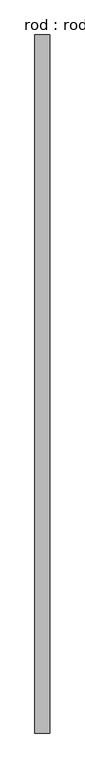
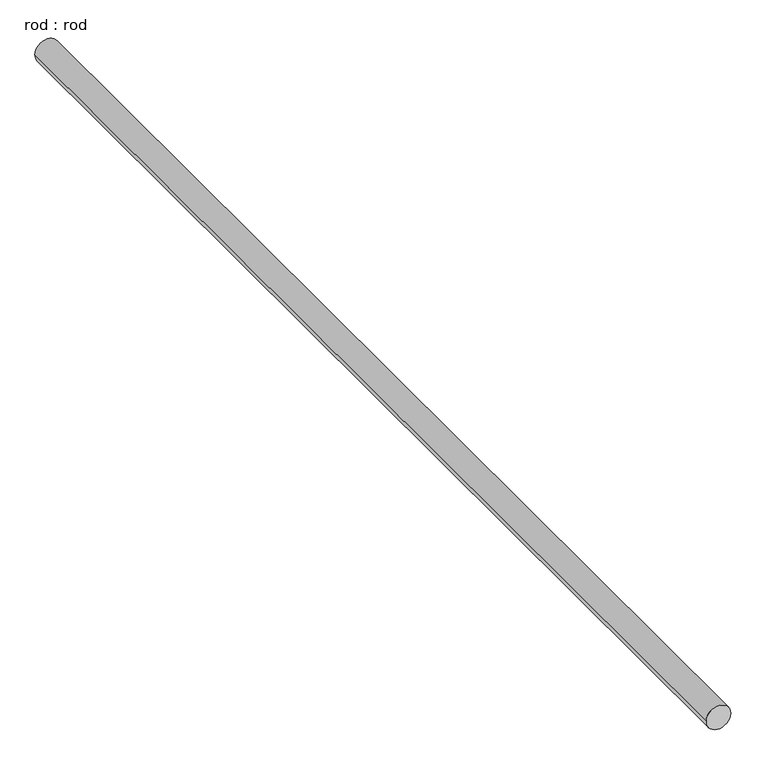
"""IFC4 building model written with IfcOpenShell, lengths in millimetres: proxy geometry, rod : rod."""

from ifc_helpers import new_model, si_unit, point, frame, frame_2d, origin, place, context, project, spatial, circle_curve, trimmed, segment, composite_curve, outline, extrude, source, transform, mapped, element, save


def rod_rod_b080d421(model_context):
    return source(origin(), model_context, "Body", "SweptSolid", [
        extrude(outline(composite_curve([segment(trimmed(circle_curve(frame_2d((0.0108462, 0.0)), 200.0), [point((0.0108462, 200.0))], [point((0.0108462, -200.0))], False, "CARTESIAN"), True, "CONTINUOUS"), segment(trimmed(circle_curve(frame_2d((0.0108462, 0.0)), 200.0), [point((0.0108462, -200.0))], [point((0.0108462, 200.0))], False, "CARTESIAN"), True, "CONTINUOUS")], self_intersect=False)), frame((0.0, -5341.9749439, 0.0), z_axis=(0.0, 1.0, 0.0), x_axis=(0.0, 0.0, 1.0)), (0.0, 0.0, 1.0), 18869.4071184),
    ])


if __name__ == "__main__":
    model = new_model("IFC4")
    model_context = context("Model", 3, world=origin())
    ifc_project = project(units=[si_unit("LENGTHUNIT", "METRE", prefix="MILLI")], contexts=[model_context])
    site = spatial("IfcSite", under=ifc_project)
    building = spatial("IfcBuilding", under=site)
    placement = place(None, origin())
    rod_rod_shape = rod_rod_b080d421(model_context)
    element("IfcBuildingElementProxy", 1, Name="rod : rod", ObjectType="rod : rod", at=placement, inside=building, context=model_context, shape_type="MappedRepresentation", body=[
        mapped(rod_rod_shape, transform((0.0, 0.0, 0.0), x_axis=(1.0, 0.0, 0.0), y_axis=(0.0, 1.0, 0.0), z_axis=(0.0, 0.0, 1.0))),
    ])
    save(model, "model.ifc")

# Revit data of these elements
# Type "rod : rod"
#   Default Elevation = 0
